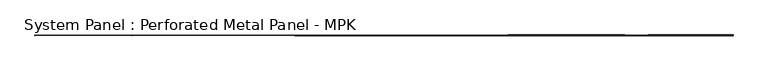
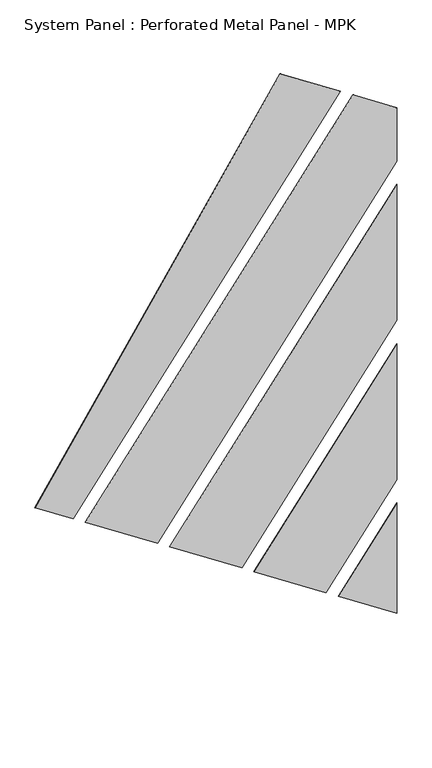
"""IFC4 building model written with IfcOpenShell, lengths in millimetres: plate geometry, System Panel : Perforated Metal Panel - MPK."""

from ifc_helpers import new_model, si_unit, frame, origin, place, context, project, spatial, polyline, outline, extrude, source, transform, mapped, element, save


def system_panel_perforated_metal_panel_mpk_dbcede24(model_context):
    return source(origin(), model_context, "Body", "SweptSolid", [
        extrude(outline(polyline([(2659.2774582, 8492.4699444), (0.0, 12533.2512196), (8060.1335901, 12533.2512196), (2659.2774582, 8492.4699444)])), frame((0.0, 0.0, 0.0), z_axis=(0.0, 1.0, 0.0), x_axis=(0.0, 0.0, 1.0)), (0.0, 0.0, 1.0), 20.0),
        extrude(outline(polyline([(16496.5090545, -12533.2512196), (14766.0852816, -9903.8663249), (39552.7658936, 8640.8888851), (42308.3486088, 4453.7714396), (16496.5090545, -12533.2512196)])), frame((0.0, 0.0, 0.0), z_axis=(0.0, 1.0, 0.0), x_axis=(0.0, 0.0, 1.0)), (0.0, 0.0, 1.0), 20.0),
        extrude(outline(polyline([(14203.8559644, -9049.5569371), (10917.8924462, -4056.524031), (33091.572061, 12533.2512196), (36991.1643838, 12533.2512196), (38990.5365764, 9495.1982729), (14203.8559644, -9049.5569371)])), frame((0.0, 0.0, 0.0), z_axis=(0.0, 1.0, 0.0), x_axis=(0.0, 0.0, 1.0)), (0.0, 0.0, 1.0), 20.0),
        extrude(outline(polyline([(10355.663129, -3202.2146433), (7069.6996108, 1790.8182628), (21427.8969383, 12533.2512196), (31387.4838355, 12533.2512196), (10355.663129, -3202.2146433)])), frame((0.0, 0.0, 0.0), z_axis=(0.0, 1.0, 0.0), x_axis=(0.0, 0.0, 1.0)), (0.0, 0.0, 1.0), 20.0),
        extrude(outline(polyline([(6507.4702936, 2645.1276506), (3221.5067754, 7638.1605567), (9764.2218156, 12533.2512196), (19723.8087128, 12533.2512196), (6507.4702936, 2645.1276506)])), frame((0.0, 0.0, 0.0), z_axis=(0.0, 1.0, 0.0), x_axis=(0.0, 0.0, 1.0)), (0.0, 0.0, 1.0), 20.0),
    ])


if __name__ == "__main__":
    model = new_model("IFC4")
    model_context = context("Model", 3, world=origin())
    ifc_project = project(units=[si_unit("LENGTHUNIT", "METRE", prefix="MILLI")], contexts=[model_context])
    site = spatial("IfcSite", under=ifc_project)
    building = spatial("IfcBuilding", under=site)
    placement = place(None, origin())
    system_panel_perforated_metal_panel_mpk_shape = system_panel_perforated_metal_panel_mpk_dbcede24(model_context)
    element("IfcPlate", 1, ObjectType="System Panel : Perforated Metal Panel - MPK", at=placement, inside=building, context=model_context, shape_type="MappedRepresentation", body=[
        mapped(system_panel_perforated_metal_panel_mpk_shape, transform((0.0, 0.0, 0.0), x_axis=(1.0, 0.0, 0.0), y_axis=(0.0, 1.0, 0.0), z_axis=(0.0, 0.0, 1.0))),
    ])
    save(model, "model.ifc")

# Revit data of these elements
# Element 1 (IfcPlate, "System Panel : Perforated Metal Panel - MPK")
#   Materials on its faces: "Perforated  Metal Panels - MPK"
# Materials
#   "Perforated  Metal Panels - MPK": class "Miscellaneous", colour RGB 127 127 127, transparency 0
